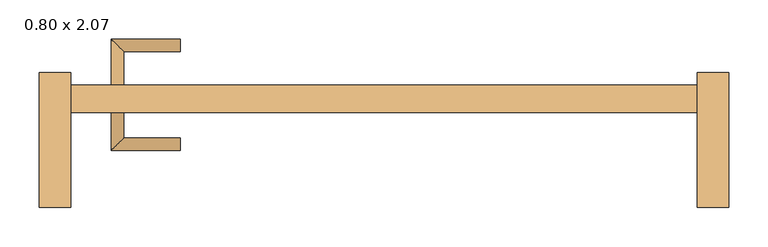
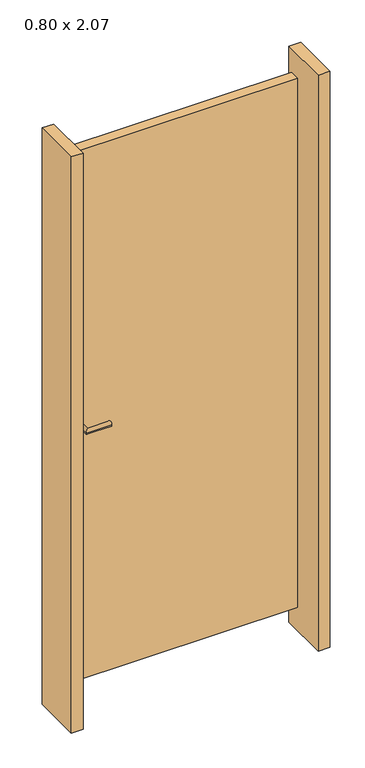
"""IFC4 building model written with IfcOpenShell, lengths in millimetres: door geometry, CC_ND 200_PORTÃO_V2018 : 0.80 x 2.07."""

import ifcopenshell
import ifcopenshell.guid

model = None  # the IFC model being written
_history = None  # IfcOwnerHistory: only IFC2X3 demands one
_inside = {}  # id of a spatial element -> (the spatial element, [elements in it])
_under = {}  # id of a project, library or spatial element -> (it, [spatial elements below it])
_declared = {}  # id of a project -> (the project, [libraries it declares])
_typed = {}  # id of a type object -> (the type object, [elements of that type])
_made_of = {}  # id of a material, layer set ... -> (it, [elements and type objects made of it])


def new_model(schema):
    """Start an empty IFC model of exactly this schema.

    Asked for "IFC4X3", IfcOpenShell would pick the latest addendum, in which some entities
    have other attributes; the version numbers below select the first issue.
    IFC2X3 requires an IfcOwnerHistory on every rooted entity: one is made here for all.
    """
    global model, _history
    if schema == "IFC4X3":
        model = ifcopenshell.file(schema_version=(4, 3, 0, 0))
    else:
        model = ifcopenshell.file(schema=schema)
    _inside.clear()
    _under.clear()
    _declared.clear()
    _typed.clear()
    _made_of.clear()
    _history = None
    if model.schema == "IFC2X3":
        org = make("IfcOrganization", Name="unknown")
        user = make(
            "IfcPersonAndOrganization",
            ThePerson=make("IfcPerson", FamilyName="unknown"),
            TheOrganization=org,
        )
        app = make(
            "IfcApplication",
            ApplicationDeveloper=org,
            Version="unknown",
            ApplicationFullName="unknown",
            ApplicationIdentifier="unknown",
        )
        _history = make(
            "IfcOwnerHistory",
            OwningUser=user,
            OwningApplication=app,
            ChangeAction="ADDED",
            CreationDate=0,
        )
    return model


def make(cls, **values):
    """One entity of the class cls with the attributes given. An attribute that is None is left unset."""
    return model.create_entity(
        cls, **{name: value for name, value in values.items() if value is not None}
    )


def rooted(cls, **values):
    """An entity with a GlobalId (a new one), such as an element, a storey or a relation."""
    return make(cls, GlobalId=ifcopenshell.guid.new(), OwnerHistory=_history, **values)


def si_unit(unit_type, name, prefix=None):
    """IfcSIUnit, for example si_unit("LENGTHUNIT", "METRE", prefix="MILLI")."""
    return make("IfcSIUnit", UnitType=unit_type, Prefix=prefix, Name=name)


def assignment(units):
    """IfcUnitAssignment: the units of a project."""
    return None if units is None else make("IfcUnitAssignment", Units=units)


def point(xyz):
    """IfcCartesianPoint."""
    return None if xyz is None else make("IfcCartesianPoint", Coordinates=xyz)


def direction(xyz):
    """IfcDirection."""
    return None if xyz is None else make("IfcDirection", DirectionRatios=xyz)


def frame(location, z_axis=None, x_axis=None):
    """IfcAxis2Placement3D, a coordinate frame: its origin and axes. An axis left out is left unset."""
    return make(
        "IfcAxis2Placement3D",
        Location=point(location),
        Axis=direction(z_axis),
        RefDirection=direction(x_axis),
    )


def origin():
    """The frame at (0, 0, 0) with its axes left unset."""
    return frame((0.0, 0.0, 0.0))


def origin_with_axes():
    """The frame at (0, 0, 0) with the z axis (0, 0, 1) and the x axis (1, 0, 0) written out."""
    return frame((0.0, 0.0, 0.0), z_axis=(0.0, 0.0, 1.0), x_axis=(1.0, 0.0, 0.0))


def place(relative_to, where):
    """IfcLocalPlacement: puts the frame where relative to a parent placement (None: the world)."""
    return make(
        "IfcLocalPlacement", PlacementRelTo=relative_to, RelativePlacement=where
    )


def context(
    kind, dimensions, precision=None, world=None, true_north=None, identifier=None
):
    """IfcGeometricRepresentationContext, for example the 3D "Model" context."""
    return make(
        "IfcGeometricRepresentationContext",
        ContextIdentifier=identifier,
        ContextType=kind,
        CoordinateSpaceDimension=dimensions,
        Precision=precision,
        WorldCoordinateSystem=world,
        TrueNorth=true_north,
    )


def project(units=None, contexts=None):
    """IfcProject with its units and contexts."""
    return rooted(
        "IfcProject",
        Name="project",
        RepresentationContexts=contexts,
        UnitsInContext=assignment(units),
    )


def spatial(cls, under=None, at=None, **own):
    """A site, building, storey or space (cls), placed at a placement, below another one or the project."""
    s = rooted(cls, ObjectPlacement=at, **own)
    if under is not None:
        _under.setdefault(under.id(), (under, []))[1].append(s)
    return s


def polyline(points):
    """IfcPolyline through the points."""
    return make("IfcPolyline", Points=[point(p) for p in points])


def circle_curve(where, radius):
    """IfcCircle in the frame where."""
    return make("IfcCircle", Position=where, Radius=radius)


def ellipse_curve(where, semi_axis1, semi_axis2):
    """IfcEllipse in the frame where."""
    return make(
        "IfcEllipse", Position=where, SemiAxis1=semi_axis1, SemiAxis2=semi_axis2
    )


def outline(outer, holes=None, kind="AREA"):
    """IfcArbitraryClosedProfileDef: a profile drawn as a closed curve; with holes, ...WithVoids."""
    if holes is None:
        return make("IfcArbitraryClosedProfileDef", ProfileType=kind, OuterCurve=outer)
    return make(
        "IfcArbitraryProfileDefWithVoids",
        ProfileType=kind,
        OuterCurve=outer,
        InnerCurves=holes,
    )


def extrude(swept, where, along, depth):
    """IfcExtrudedAreaSolid: the profile swept, set in the frame where, extruded along a direction by depth."""
    return make(
        "IfcExtrudedAreaSolid",
        SweptArea=swept,
        Position=where,
        ExtrudedDirection=direction(along),
        Depth=depth,
    )


def shape(context_of_items, identifier, shape_type, items):
    """IfcShapeRepresentation: the items that make up one representation, for example the "Body"."""
    return make(
        "IfcShapeRepresentation",
        ContextOfItems=context_of_items,
        RepresentationIdentifier=identifier,
        RepresentationType=shape_type,
        Items=items,
    )


def source(mapping_origin, context_of_items, identifier, shape_type, items):
    """IfcRepresentationMap: a shape defined once, which mapped items show again and again."""
    return make(
        "IfcRepresentationMap",
        MappingOrigin=mapping_origin,
        MappedRepresentation=shape(context_of_items, identifier, shape_type, items),
    )


def transform(
    local_origin,
    x_axis=None,
    y_axis=None,
    z_axis=None,
    scale=None,
    scale2=None,
    scale3=None,
    uniform=True,
):
    """IfcCartesianTransformationOperator3D, or its non-uniform kind. x_axis, y_axis, z_axis: its Axis1, 2, 3."""
    if uniform:
        return make(
            "IfcCartesianTransformationOperator3D",
            Axis1=direction(x_axis),
            Axis2=direction(y_axis),
            LocalOrigin=point(local_origin),
            Scale=scale,
            Axis3=direction(z_axis),
        )
    return make(
        "IfcCartesianTransformationOperator3DnonUniform",
        Axis1=direction(x_axis),
        Axis2=direction(y_axis),
        LocalOrigin=point(local_origin),
        Scale=scale,
        Axis3=direction(z_axis),
        Scale2=scale2,
        Scale3=scale3,
    )


def mapped(mapping_source, mapping_target):
    """IfcMappedItem: shows the shape of a source again, moved by a transform."""
    return make(
        "IfcMappedItem", MappingSource=mapping_source, MappingTarget=mapping_target
    )


def made_of(thing, what):
    """Note that an element or type object is made of a material, layer set ...; save() writes the relation."""
    if what is not None:
        _made_of.setdefault(what.id(), (what, []))[1].append(thing)
    return thing


def element(
    cls,
    number,
    at=None,
    inside=None,
    cuts=None,
    type_object=None,
    material=None,
    context=None,
    identifier="Body",
    shape_type=None,
    held_by="IfcProductDefinitionShape",
    body=None,
    shapes=None,
    **own,
):
    """One element of the class cls, such as IfcWall. Its Tag is "e" and its number.

    at: its placement. inside: the storey or other place that contains it. cuts: it is an
    opening in that element (IfcRelVoidsElement). A single representation is given by context,
    identifier, shape_type and body (its items); several are given by shapes. held_by: the class
    of the entity that holds the representations. save() writes the other relations.
    """
    e = rooted(cls, Tag="e%d" % number, ObjectPlacement=at, **own)
    if body is not None:
        shapes = [shape(context, identifier, shape_type, body)]
    if shapes is not None:
        e.Representation = make(held_by, Representations=shapes)
    if inside is not None:
        _inside.setdefault(inside.id(), (inside, []))[1].append(e)
    if cuts is not None:
        rooted(
            "IfcRelVoidsElement", RelatingBuildingElement=cuts, RelatedOpeningElement=e
        )
    if type_object is not None:
        _typed.setdefault(type_object.id(), (type_object, []))[1].append(e)
    return made_of(e, material)


def aggregate(whole, parts):
    """IfcRelAggregates: a whole, such as a stair, and the parts it consists of."""
    return rooted("IfcRelAggregates", RelatingObject=whole, RelatedObjects=parts)


def save(model, path):
    """Write the relations noted so far, then the file.

    IfcRelAggregates (storeys below a building ...), IfcRelContainedInSpatialStructure (elements
    in a storey), IfcRelDefinesByType, IfcRelAssociatesMaterial and IfcRelDeclares: one each for
    every whole, place, type object, material and project.
    """
    for whole, parts in _under.values():
        aggregate(whole, parts)
    for where, things in _inside.values():
        rooted(
            "IfcRelContainedInSpatialStructure",
            RelatedElements=things,
            RelatingStructure=where,
        )
    for kind, things in _typed.values():
        rooted("IfcRelDefinesByType", RelatedObjects=things, RelatingType=kind)
    for what, things in _made_of.values():
        rooted("IfcRelAssociatesMaterial", RelatedObjects=things, RelatingMaterial=what)
    for by, libraries in _declared.values():
        rooted("IfcRelDeclares", RelatingContext=by, RelatedDefinitions=libraries)
    model.write(path)


def plane_surface(at):
    """IfcPlane: the flat surface through the origin of the frame at, square to its z axis."""
    return make("IfcPlane", Position=at)


def cylinder_surface(at, radius):
    """IfcCylindricalSurface: all points at the distance radius from the z axis of the frame at."""
    return make("IfcCylindricalSurface", Position=at, Radius=radius)


def advanced_brep(points, edges, surfaces, faces):
    """IfcAdvancedBrep: a solid bounded by faces that lie on surfaces and meet in shared edges.

    An edge is (start, end): straight between two places in points (the first is 0);
    or (start, end, curve); or (start, end, curve, False) where it runs against its curve.
    A face is (place in surfaces, loops), or (place, loops, False) where it looks against
    its surface's normal. A loop lists edges by number (the first is 1), with a minus sign
    where the edge is run from its end to its start. The first loop is the outer one.
    """
    corners = [point(p) for p in points]
    vertices = [make("IfcVertexPoint", VertexGeometry=c) for c in corners]
    made = []
    for start, end, *more in edges:
        made.append(
            make(
                "IfcEdgeCurve",
                EdgeStart=vertices[start],
                EdgeEnd=vertices[end],
                EdgeGeometry=more[0] if more else make("IfcPolyline", Points=[corners[start], corners[end]]),
                SameSense=more[1] if len(more) > 1 else True,
            )
        )
    hull = []
    for where, loops, *sense in faces:
        bounds = []
        for j, loop in enumerate(loops):
            ring = [make("IfcOrientedEdge", EdgeElement=made[abs(k) - 1], Orientation=k > 0) for k in loop]
            bounds.append(
                make(
                    "IfcFaceOuterBound" if j == 0 else "IfcFaceBound",
                    Bound=make("IfcEdgeLoop", EdgeList=ring),
                    Orientation=True,
                )
            )
        hull.append(make("IfcAdvancedFace", Bounds=bounds, FaceSurface=surfaces[where], SameSense=sense[0] if sense else True))
    return make("IfcAdvancedBrep", Outer=make("IfcClosedShell", CfsFaces=hull))


def door_0_80_x_2_07_c914aa4f(model_context):
    return source(origin(), model_context, "Body", "SolidModel", [
        advanced_brep(
        [(-348.0, 70.0, 1000.0), (-332.0, 70.0, 1000.0), (-348.0, 129.0, 1000.0), (-332.0, 113.0, 1000.0), (-260.0, 129.0, 1000.0), (-260.0, 113.0, 1000.0)],
        [
            (0, 1, circle_curve(frame((-340.0, 70.0, 1000.0), z_axis=(0.0, -1.0, 0.0), x_axis=(1.0, 0.0, 0.0)), 8.0)),
            (1, 0, circle_curve(frame((-340.0, 70.0, 1000.0), z_axis=(0.0, -1.0, 0.0), x_axis=(1.0, 0.0, 0.0)), 8.0)),
            (0, 2),
            (2, 3, ellipse_curve(frame((-340.0, 121.0, 1000.0), z_axis=(-0.707106781186538, -0.707106781186557, 0.0), x_axis=(0.707106781186557, -0.707106781186538, 0.0)), 11.3137085, 8.0)),
            (3, 1),
            (3, 2, ellipse_curve(frame((-340.0, 121.0, 1000.0), z_axis=(-0.707106781186538, -0.707106781186557, 0.0), x_axis=(0.707106781186557, -0.707106781186538, 0.0)), 11.3137085, 8.0)),
            (4, 5, circle_curve(frame((-260.0, 121.0, 1000.0), z_axis=(1.0, 0.0, 0.0), x_axis=(0.0, -1.0, 0.0)), 8.0)),
            (5, 4, circle_curve(frame((-260.0, 121.0, 1000.0), z_axis=(1.0, 0.0, 0.0), x_axis=(0.0, -1.0, 0.0)), 8.0)),
            (2, 4),
            (5, 3),
        ],
        [
            plane_surface(frame((-340.0, 70.0, 0.0), z_axis=(0.0, -1.0, 0.0), x_axis=(0.0, 0.0, 1.0))),
            cylinder_surface(frame((-340.0, 70.0, 1000.0), z_axis=(0.0, -1.0, 0.0), x_axis=(1.0, 0.0, 0.0)), 8.0),
            plane_surface(frame((-260.0, 121.0, 0.0), z_axis=(1.0, 0.0, 0.0), x_axis=(0.0, 0.0, 1.0))),
            cylinder_surface(frame((-340.0, 121.0, 1000.0), z_axis=(-1.0, 0.0, 0.0), x_axis=(0.0, -1.0, 0.0)), 8.0),
        ],
        [
            (0, [[1, 2]]),
            (1, [[3, 4, 5, -1]]),
            (1, [[-5, 6, -3, -2]]),
            (2, [[7, 8]]),
            (3, [[9, -8, 10, -4]]),
            (3, [[-10, -7, -9, -6]]),
        ],
    ),
        advanced_brep(
        [(-332.0, 35.0, 1000.0), (-348.0, 35.0, 1000.0), (-348.0, -13.0, 1000.0), (-332.0, 3.0, 1000.0), (-260.0, 3.0, 1000.0), (-260.0, -13.0, 1000.0)],
        [
            (0, 1, circle_curve(frame((-340.0, 35.0, 1000.0), z_axis=(0.0, 1.0, 0.0), x_axis=(-1.0, 0.0, 0.0)), 8.0)),
            (1, 0, circle_curve(frame((-340.0, 35.0, 1000.0), z_axis=(0.0, 1.0, 0.0), x_axis=(-1.0, 0.0, 0.0)), 8.0)),
            (1, 2),
            (2, 3, ellipse_curve(frame((-340.0, -5.0, 1000.0), z_axis=(-0.7071067811865475, 0.7071067811865475, 0.0), x_axis=(0.7071067811865474, 0.7071067811865476, 0.0)), 11.3137085, 8.0)),
            (3, 0),
            (3, 2, ellipse_curve(frame((-340.0, -5.0, 1000.0), z_axis=(-0.7071067811865475, 0.7071067811865475, 0.0), x_axis=(0.7071067811865474, 0.7071067811865476, 0.0)), 11.3137085, 8.0)),
            (4, 5, circle_curve(frame((-260.0, -5.0, 1000.0), z_axis=(1.0, 0.0, 0.0), x_axis=(0.0, -1.0, 0.0)), 8.0)),
            (5, 4, circle_curve(frame((-260.0, -5.0, 1000.0), z_axis=(1.0, 0.0, 0.0), x_axis=(0.0, -1.0, 0.0)), 8.0)),
            (2, 5),
            (4, 3),
        ],
        [
            plane_surface(frame((-340.0, 35.0, 0.0), z_axis=(0.0, 1.0, 0.0), x_axis=(0.0, 0.0, 1.0))),
            cylinder_surface(frame((-340.0, 35.0, 1000.0), z_axis=(0.0, 1.0, 0.0), x_axis=(-1.0, 0.0, 0.0)), 8.0),
            plane_surface(frame((-260.0, -5.0, 0.0), z_axis=(1.0, 0.0, 0.0), x_axis=(0.0, 0.0, 1.0))),
            cylinder_surface(frame((-340.0, -5.0, 1000.0), z_axis=(-1.0, 0.0, 0.0), x_axis=(0.0, -1.0, 0.0)), 8.0),
        ],
        [
            (0, [[1, 2]]),
            (1, [[3, 4, 5, -2]]),
            (1, [[-5, 6, -3, -1]]),
            (2, [[7, 8]]),
            (3, [[9, -7, 10, -4]]),
            (3, [[-10, -8, -9, -6]]),
        ],
    ),
        extrude(outline(polyline([(400.0, 70.0), (400.0, 35.0), (-400.0, 35.0), (-400.0, 70.0), (400.0, 70.0)])), frame((0.0, 0.0, 85.0), z_axis=(0.0, 0.0, 1.0), x_axis=(1.0, 0.0, 0.0)), (0.0, 0.0, 1.0), 1900.0),
        extrude(outline(polyline([(-440.0, -86.0), (-440.0, 86.0), (-400.0, 86.0), (-400.0, -86.0), (-440.0, -86.0)])), origin_with_axes(), (0.0, 0.0, 1.0), 2070.0),
        extrude(outline(polyline([(440.0, -86.0), (400.0, -86.0), (400.0, 86.0), (440.0, 86.0), (440.0, -86.0)])), origin_with_axes(), (0.0, 0.0, 1.0), 2070.0),
    ])


if __name__ == "__main__":
    model = new_model("IFC4")
    model_context = context("Model", 3, world=origin())
    ifc_project = project(units=[si_unit("LENGTHUNIT", "METRE", prefix="MILLI")], contexts=[model_context])
    site = spatial("IfcSite", under=ifc_project)
    building = spatial("IfcBuilding", under=site)
    placement = place(None, origin())
    door_0_80_x_2_07_shape = door_0_80_x_2_07_c914aa4f(model_context)
    element("IfcDoor", 1, ObjectType="CC_ND 200_PORTÃO_V2018 : 0.80 x 2.07", at=placement, inside=building, context=model_context, shape_type="MappedRepresentation", body=[
        mapped(door_0_80_x_2_07_shape, transform((0.0, 0.0, 0.0), x_axis=(1.0, 0.0, 0.0), y_axis=(0.0, 1.0, 0.0), z_axis=(0.0, 0.0, 1.0))),
    ])
    save(model, "model.ifc")

# Revit data of these elements
# Project information
#   Design Option = "Main Model"
#   Project Status = "Status do projeto"
#   Project Address = "RUA SÉRGIO DIAS, LOTE 30, QUADRA G, MONTE MINEIRO/MG"
#   Project Name = "RESIDÊNCIA - ROBERTA VENDRAMINI"
#   Project Number = "034/2017"
#   Zona = "ZER - 01"
#   CA Mín = "0.2"
#   CA Básico = "1"
#   CA Máx = "2"
#   TO Máx = "50"
#   Gabarito Máx = "10"
#   TP Mín = "15"
#   Área Total do Terreno = "620.00 m²"
#   Multifamiliar - Vagas Veículos/Pavto = "0"
#   Multifamiliar - Vagas Bicicletas/Pavto = "0"
#   Multifamiliar - % Vagas PNMR = "0"
#   Multifamiliar - % Vagas Motos = "0"
#   Outros - Área p/ 1 Veículo = "0.00 m²"
#   Outros - Área p/ 1 Bicicleta = "0.00 m²"
#   Outros - Área p/ 1 Utilitário = "0.00 m²"
#   Outros - % Vagas PNMR = "0"
#   Outros - % Vagas Motos = "0"
# Type "CC_ND 200_PORTÃO_V2018 : 0.80 x 2.07"
#   Type Mark = "141"
#   Analytic Construction = "<Nenhum>"
#   Vão superior = 0.085 m
#   Vão inferior = 0.085 m
#   Largura_moldura = 0.08 m
#   Espessura_moldura = 0.01 m
#   Espessura_batente = 0.04 m
#   Thickness = 0.05 m
#   Altura do portão = 1.90 m
#   Rough Width = 0.88 m
#   Rough Height = 1.73 m
#   Height = 1.73 m
#   Width = 0.80 m
#   Soleira [instance default] = no
#   Moldura_interna [instance default] = no
#   Moldura_externa [instance default] = no
#   Maçaneta [instance default] = no
#   Acabamento moldura [instance default] = none
#   Acabamento batente [instance default] = none
#   Acabamento maçaneta [instance default] = none
#   Acabamento folha da porta [instance default] = none
#   Acabamento soleira [instance default] = none
#   Function = (empty or 0)
#   Wall Closure = (empty or 0)
# Element 1 (IfcDoor, "CC_ND 200_PORTÃO_V2018 : 0.80 x 2.07")
#   Maçaneta = yes
#   Acabamento moldura = .ALUMÍNIO
#   Acabamento batente = .MADEIRA_CEREJEIRA CLARO
#   Acabamento folha da porta = .MADEIRA_CEREJEIRA CLARO
#   Materials on its faces: ".MADEIRA_CEREJEIRA CLARO"
# Materials
#   ".MADEIRA_CEREJEIRA CLARO": class ".CC_MADEIRA REVEST.", colour RGB 233 182 144, transparency 0, Cost = 0
#   ".ALUMÍNIO": class "CC_METAIS", colour RGB 244 244 244, transparency 0, Description = "Material alumínio", Cost = 0
